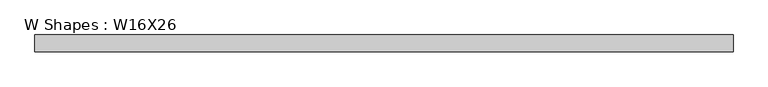
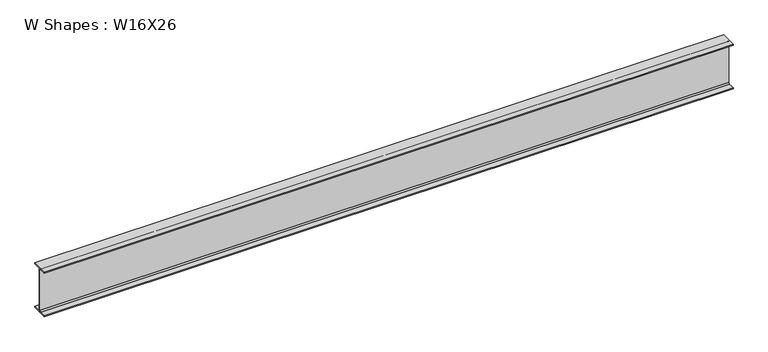
"""IFC4 building model written with IfcOpenShell, lengths in millimetres: beam geometry, W Shapes : W16X26."""

from ifc_helpers import new_model, si_unit, point, frame, frame_2d, origin, place, context, project, spatial, polyline, circle_curve, trimmed, segment, composite_curve, outline, extrude, source, transform, mapped, element, save


def w_shapes_w16x26_f77c1278(model_context):
    return source(origin(), model_context, "Body", "SweptSolid", [
        extrude(outline(composite_curve([segment(polyline([(69.85, -190.627), (69.85, -199.39), (-69.85, -199.39), (-69.85, -190.627), (-13.3858, -190.627)]), True, "CONTINUOUS"), segment(trimmed(circle_curve(frame_2d((-13.3858, -180.4162)), 10.2108), [point((-13.3858, -190.627))], [point((-3.175, -180.4162))], True, "CARTESIAN"), True, "CONTINUOUS"), segment(polyline([(-3.175, -180.4162), (-3.175, 180.4162)]), True, "CONTINUOUS"), segment(trimmed(circle_curve(frame_2d((-13.3858, 180.4162)), 10.2108), [point((-3.175, 180.4162))], [point((-13.3858, 190.627))], True, "CARTESIAN"), True, "CONTINUOUS"), segment(polyline([(-13.3858, 190.627), (-69.85, 190.627), (-69.85, 199.39), (69.85, 199.39), (69.85, 190.627), (13.3858, 190.627)]), True, "CONTINUOUS"), segment(trimmed(circle_curve(frame_2d((13.3858, 180.4162)), 10.2108), [point((13.3858, 190.627))], [point((3.175, 180.4162))], True, "CARTESIAN"), True, "CONTINUOUS"), segment(polyline([(3.175, 180.4162), (3.175, -180.4162)]), True, "CONTINUOUS"), segment(trimmed(circle_curve(frame_2d((13.3858, -180.4162)), 10.2108), [point((3.175, -180.4162))], [point((13.3858, -190.627))], True, "CARTESIAN"), True, "CONTINUOUS"), segment(polyline([(13.3858, -190.627), (69.85, -190.627)]), True, "CONTINUOUS")], self_intersect=False)), frame((-2921.0, 0.0, 0.0), z_axis=(1.0, 0.0, 0.0), x_axis=(0.0, 1.0, 0.0)), (0.0, 0.0, 1.0), 5842.0),
    ])


if __name__ == "__main__":
    model = new_model("IFC4")
    model_context = context("Model", 3, world=origin())
    ifc_project = project(units=[si_unit("LENGTHUNIT", "METRE", prefix="MILLI")], contexts=[model_context])
    site = spatial("IfcSite", under=ifc_project)
    building = spatial("IfcBuilding", under=site)
    placement = place(None, origin())
    w_shapes_w16x26_shape = w_shapes_w16x26_f77c1278(model_context)
    element("IfcBeam", 1, ObjectType="W Shapes : W16X26", at=placement, inside=building, context=model_context, shape_type="MappedRepresentation", body=[
        mapped(w_shapes_w16x26_shape, transform((0.0, 0.0, 0.0), x_axis=(1.0, 0.0, 0.0), y_axis=(0.0, 1.0, 0.0), z_axis=(0.0, 0.0, 1.0))),
    ])
    save(model, "model.ifc")

# Revit data of these elements
# Type "W Shapes : W16X26"
#   Section Name Key = "W16x26"
#   Assembly Code = "B10"
#   Width = 5.500"
#   Web Thickness = 0.250"
#   Web Fillet = 0.402"
#   Warping Constant = 565.00 in⁶
#   Torsional Moment of Inertia = 0.262 in⁴
#   Section Area = 7.68 in²
#   Plastic Modulus weak axis = 5.48 in³
#   Plastic Modulus strong axis = 44.20 in³
#   Perimeter = 4.35 ft²/ft
#   Nominal Weight = 26.00 lbf/ft
#   Moment of Inertia weak axis = 9.59 in⁴
#   Moment of Inertia strong axis = 301.00 in⁴
#   Height = 15.700"
#   Flange Thickness = 0.345"
#   Elastic Modulus weak axis = 3.49 in³
#   Elastic Modulus strong axis = 38.40 in³
#   Centroid Vertical = 7.850"
#   Centroid Horizontal = 2.750"
#   Bolt Spacing = 0' - 3 1/2"
#   Length [instance default] = 5' - 0"
#   Structural Material [instance default] = Steel ASTM A992
#   Principal Axes Angle = 0
# Element 1 (IfcBeam, "W Shapes : W16X26")
#   Structural Material = Steel ASTM A36
#   Materials on its faces: "Steel ASTM A36"
# Materials
#   "Steel ASTM A992": class "Metal", colour RGB 199 199 199, transparency 0, Description = "Structural steel 50ksi", Cost = 0
#   "Steel ASTM A36": class "Metal", colour RGB 199 199 199, transparency 0, Description = "Structural steel, ASTM A36 Grade B, mill finish", Cost = 0
